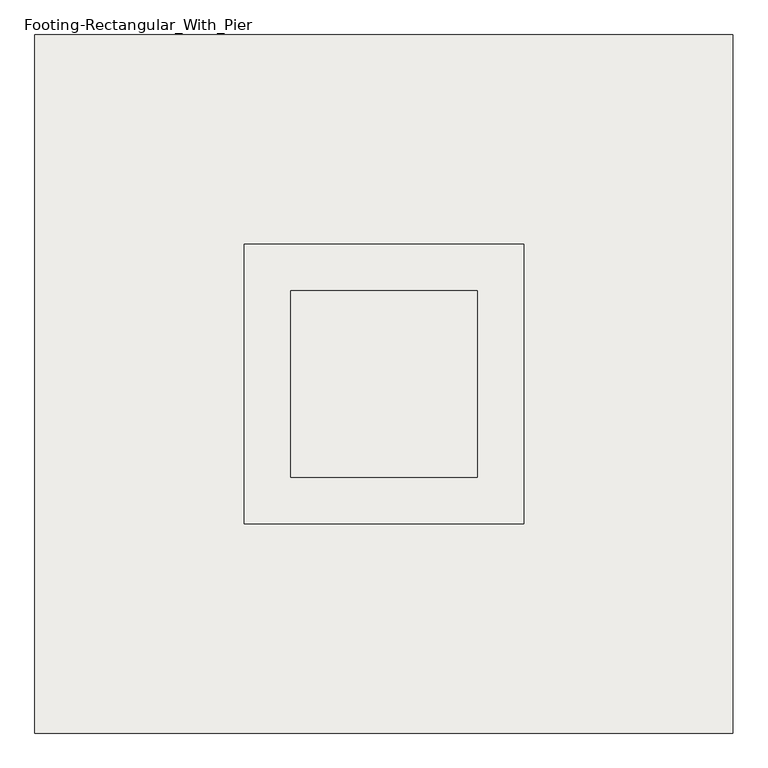
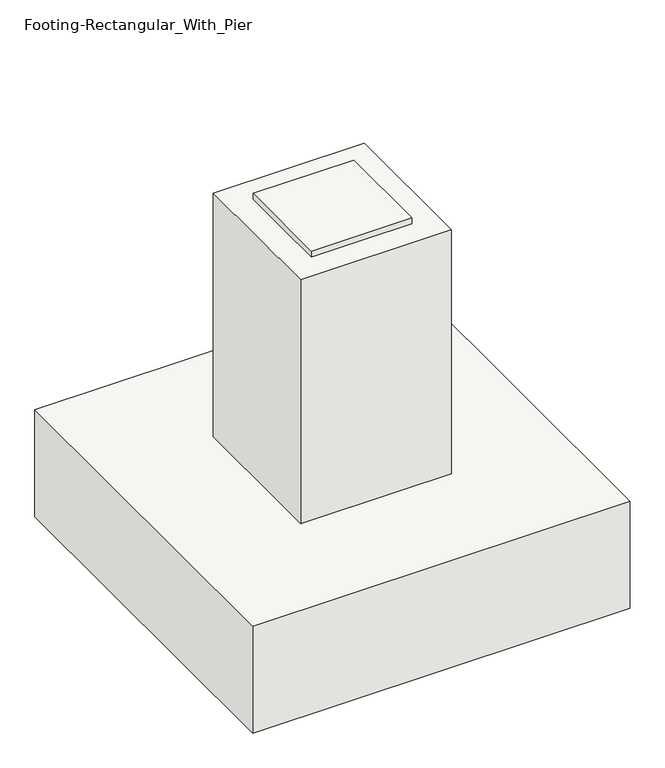
"""IFC4 building model written with IfcOpenShell, lengths in millimetres: slab geometry, Footing-Rectangular_With_Pier."""

from ifc_helpers import new_model, si_unit, frame, origin, origin_with_axes, place, context, project, spatial, polyline, outline, extrude, source, transform, mapped, element, save


def footing_rectangular_with_pier_073162b1(model_context):
    return source(origin(), model_context, "Body", "SweptSolid", [
        extrude(outline(polyline([(203.2, 203.2), (203.2, -203.2), (-203.2, -203.2), (-203.2, 203.2), (203.2, 203.2)])), frame((0.0, 0.0, 1041.4), z_axis=(0.0, 0.0, 1.0), x_axis=(1.0, 0.0, 0.0)), (0.0, 0.0, 1.0), 25.4),
        extrude(outline(polyline([(304.8, 304.8), (304.8, -304.8), (-304.8, -304.8), (-304.8, 304.8), (304.8, 304.8)])), origin_with_axes(), (0.0, 0.0, 1.0), 1041.4),
        extrude(outline(polyline([(762.0, 762.0), (762.0, -762.0), (-762.0, -762.0), (-762.0, 762.0), (762.0, 762.0)])), frame((0.0, 0.0, -457.2), z_axis=(0.0, 0.0, 1.0), x_axis=(1.0, 0.0, 0.0)), (0.0, 0.0, 1.0), 457.2),
    ])


if __name__ == "__main__":
    model = new_model("IFC4")
    model_context = context("Model", 3, world=origin())
    ifc_project = project(units=[si_unit("LENGTHUNIT", "METRE", prefix="MILLI")], contexts=[model_context])
    site = spatial("IfcSite", under=ifc_project)
    building = spatial("IfcBuilding", under=site)
    placement = place(None, origin())
    footing_rectangular_with_pier_shape = footing_rectangular_with_pier_073162b1(model_context)
    element("IfcSlab", 1, ObjectType="Footing-Rectangular_With_Pier : F8 - 5'-0\" x 5'-0\" x 1'-6\" 2", at=placement, inside=building, context=model_context, shape_type="MappedRepresentation", body=[
        mapped(footing_rectangular_with_pier_shape, transform((0.0, 0.0, 0.0), x_axis=(1.0, 0.0, 0.0), y_axis=(0.0, 1.0, 0.0), z_axis=(0.0, 0.0, 1.0))),
    ])
    save(model, "model.ifc")

# Revit data of these elements
# Type "Footing-Rectangular_With_Pier : F8 - 5'-0\" x 5'-0\" x 1'-6\" 2"
#   Assembly Code = "A1010100"
#   Width = 1524 mm
#   SteelPlateWidth [instance default] = 406.4 mm
#   SteelPlateThickness [instance default] = 25.4 mm
#   SteelPlateDepth [instance default] = 406.4 mm
#   PierWidth [instance default] = 609.6 mm
#   PierLength [instance default] = 609.6 mm
#   PierDepth [instance default] = 1371.6 mm
#   Length = 1524 mm
#   FootingThickness = 457.2 mm
#   Steel Plate = yes
#   Structural Material [instance default] = Concrete - Cast-in-Place Concrete
# Element 1 (IfcSlab, "Footing-Rectangular_With_Pier : F8 - 5'-0\" x 5'-0\" x 1'-6\" 2")
#   PierDepth = 1041.4 mm
#   Materials on its faces: "Concrete - Cast-in-Place Concrete", "Steel"
# Materials
#   "Concrete - Cast-in-Place Concrete": class "Concrete", colour RGB 192 192 192, transparency 0
#   "Steel": class "Metal", colour RGB 247 247 247, transparency 0, Description = "Steel, mill finish", Cost = 0
